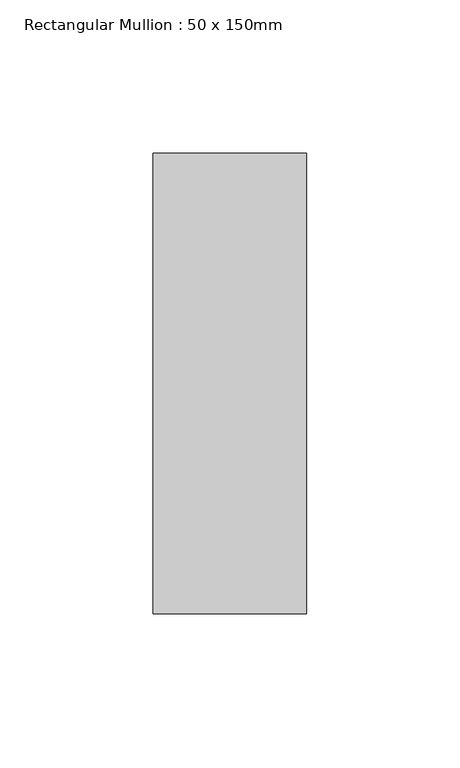
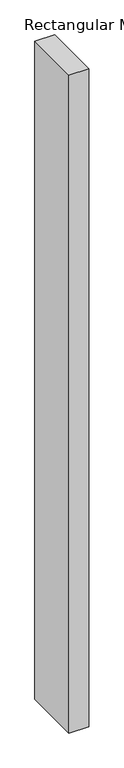
"""IFC4 building model written with IfcOpenShell, lengths in millimetres: member geometry, Rectangular Mullion : 50 x 150mm."""

from ifc_helpers import new_model, si_unit, frame, origin, place, context, project, spatial, polyline, outline, extrude, source, transform, mapped, element, save


def rectangular_mullion_50_x_150mm_41ec5d26(model_context):
    return source(origin(), model_context, "Body", "SweptSolid", [
        extrude(outline(polyline([(0.0, 75.0), (0.0, -75.0), (-50.0, -75.0), (-50.0, 75.0), (0.0, 75.0)])), frame((0.0, 0.0, -1767.0), z_axis=(0.0, 0.0, 1.0), x_axis=(1.0, 0.0, 0.0)), (0.0, 0.0, 1.0), 1767.0),
    ])


if __name__ == "__main__":
    model = new_model("IFC4")
    model_context = context("Model", 3, world=origin())
    ifc_project = project(units=[si_unit("LENGTHUNIT", "METRE", prefix="MILLI")], contexts=[model_context])
    site = spatial("IfcSite", under=ifc_project)
    building = spatial("IfcBuilding", under=site)
    placement = place(None, origin())
    rectangular_mullion_50_x_150mm_shape = rectangular_mullion_50_x_150mm_41ec5d26(model_context)
    element("IfcMember", 1, ObjectType="Rectangular Mullion : 50 x 150mm", at=placement, inside=building, context=model_context, shape_type="MappedRepresentation", body=[
        mapped(rectangular_mullion_50_x_150mm_shape, transform((0.0, 0.0, 0.0), x_axis=(1.0, 0.0, 0.0), y_axis=(0.0, 1.0, 0.0), z_axis=(0.0, 0.0, 1.0))),
    ])
    save(model, "model.ifc")

# Revit data of these elements
# Type "Rectangular Mullion : 50 x 150mm"
#   Keynote = "H11"
#   built-in parameter 1007304 = 0.492126 (stored number, unit not read)
#   built-in parameter 1007301 = 0.082021 (stored number, unit not read)
#   built-in parameter 1007300 = 0.082021 (stored number, unit not read)
# Element 1 (IfcMember, "Rectangular Mullion : 50 x 150mm")
#   Materials on its faces: "Aluminium"
# Materials
#   "Aluminium": class "Metal", colour RGB 247 247 247, transparency 0, Description = "Aluminium 6061", Cost = 0
